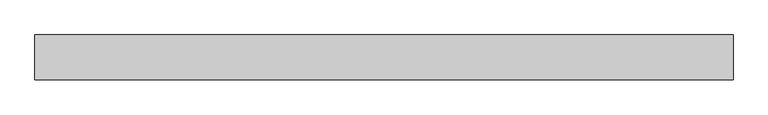
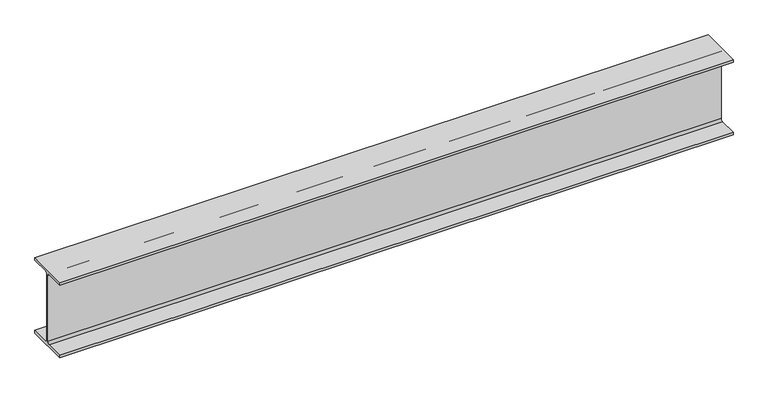
"""IFC4 building model written with IfcOpenShell, lengths in millimetres: beam geometry, Old_Steel Beam_H-KSD3502 : H_SB_ASB_H-200×200x8x12."""

from ifc_helpers import new_model, si_unit, point, frame, frame_2d, origin, place, context, project, spatial, polyline, circle_curve, trimmed, segment, composite_curve, outline, extrude, source, transform, mapped, element, save


def beam_1a68ff55(model_context):
    return source(origin(), model_context, "Body", "SweptSolid", [
        extrude(outline(composite_curve([segment(polyline([(82.5, -141.5), (82.5, -151.7), (-82.5, -151.7), (-82.5, -141.5), (-11.9, -141.5)]), True, "CONTINUOUS"), segment(trimmed(circle_curve(frame_2d((-11.9, -132.6)), 8.9), [point((-11.9, -141.5))], [point((-3.0, -132.6))], True, "CARTESIAN"), True, "CONTINUOUS"), segment(polyline([(-3.0, -132.6), (-3.0, 132.6)]), True, "CONTINUOUS"), segment(trimmed(circle_curve(frame_2d((-11.9, 132.6)), 8.9), [point((-3.0, 132.6))], [point((-11.9, 141.5))], True, "CARTESIAN"), True, "CONTINUOUS"), segment(polyline([(-11.9, 141.5), (-82.5, 141.5), (-82.5, 151.7), (82.5, 151.7), (82.5, 141.5), (11.9, 141.5)]), True, "CONTINUOUS"), segment(trimmed(circle_curve(frame_2d((11.9, 132.6)), 8.9), [point((11.9, 141.5))], [point((3.0, 132.6))], True, "CARTESIAN"), True, "CONTINUOUS"), segment(polyline([(3.0, 132.6), (3.0, -132.6)]), True, "CONTINUOUS"), segment(trimmed(circle_curve(frame_2d((11.9, -132.6)), 8.9), [point((3.0, -132.6))], [point((11.9, -141.5))], True, "CARTESIAN"), True, "CONTINUOUS"), segment(polyline([(11.9, -141.5), (82.5, -141.5)]), True, "CONTINUOUS")], self_intersect=False)), frame((-1163.5370232, 0.0, 0.0), z_axis=(1.0, 0.0, 0.0), x_axis=(0.0, 1.0, 0.0)), (0.0, 0.0, 1.0), 2569.9968936),
    ])


if __name__ == "__main__":
    model = new_model("IFC4")
    model_context = context("Model", 3, world=origin())
    ifc_project = project(units=[si_unit("LENGTHUNIT", "METRE", prefix="MILLI")], contexts=[model_context])
    site = spatial("IfcSite", under=ifc_project)
    building = spatial("IfcBuilding", under=site)
    placement = place(None, origin())
    beam_shape = beam_1a68ff55(model_context)
    element("IfcBeam", 1, ObjectType="Old_Steel Beam_H-KSD3502 : H_SB_ASB_H-200×200x8x12", at=placement, inside=building, context=model_context, shape_type="MappedRepresentation", body=[
        mapped(beam_shape, transform((0.0, 0.0, 0.0), x_axis=(1.0, 0.0, 0.0), y_axis=(0.0, 1.0, 0.0), z_axis=(0.0, 0.0, 1.0))),
    ])
    save(model, "model.ifc")

# Revit data of these elements
# Type "Old_Steel Beam_H-KSD3502 : H_SB_ASB_H-200×200x8x12"
#   Width = 20.0 cm
#   Web Thickness = 0.8 cm
#   Web Fillet = 1.3 cm
#   Warping Constant = 141376.0 cm⁶
#   Torsional Moment of Inertia = 26.2485 cm⁴
#   Torsional Modulus = 1.0 cm³
#   Section Area = 63.53 cm²
#   Plastic Modulus weak axis = 244.0 cm³
#   Plastic Modulus strong axis = 525.0 cm³
#   Perimeter = 1.16 m²/m
#   Nominal Weight = 49.90 kgf/m
#   Moment of Inertia weak axis = 1600.00 cm⁴
#   Moment of Inertia strong axis = 4720.00 cm⁴
#   Height = 20.0 cm
#   Flange Thickness = 1.2 cm
#   Elastic Modulus weak axis = 160.0 cm³
#   Elastic Modulus strong axis = 472.0 cm³
#   Centroid Vertical = 10.0 cm
#   Centroid Horizontal = 10.0 cm
#   Length [instance default] = 1.5240 m
#   Structural Material [instance default] = Steel, 45-345
#   Assembly Code = ""
# Element 1 (IfcBeam, "Old_Steel Beam_H-KSD3502 : H_SB_ASB_H-200×200x8x12")
#   Structural Material = none
# Materials
#   "Steel, 45-345": class "Metal", colour RGB 189 187 185, transparency 0, Description = "Steel 345 MPa", Cost = 0
